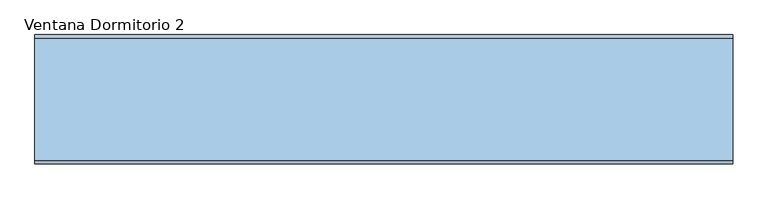
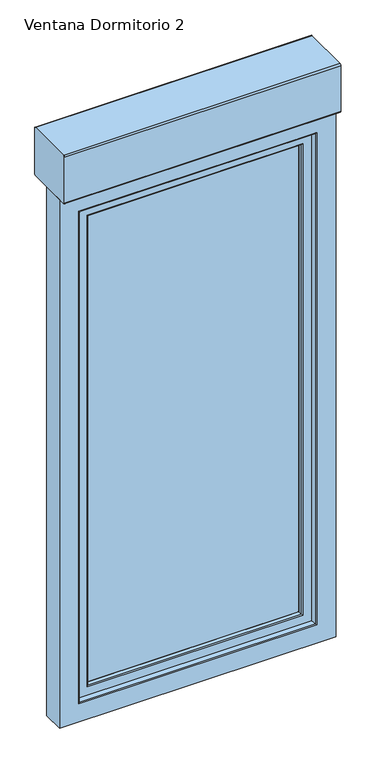
"""IFC4 building model written with IfcOpenShell, lengths in millimetres: window geometry, 2019_ES_Ventana_Replus_re80pvc301_10100_box_1-Hoja_con-Compacto : Ventana Dormitorio 2."""

import ifcopenshell
import ifcopenshell.guid

model = None  # the IFC model being written
_history = None  # IfcOwnerHistory: only IFC2X3 demands one
_inside = {}  # id of a spatial element -> (the spatial element, [elements in it])
_under = {}  # id of a project, library or spatial element -> (it, [spatial elements below it])
_declared = {}  # id of a project -> (the project, [libraries it declares])
_typed = {}  # id of a type object -> (the type object, [elements of that type])
_made_of = {}  # id of a material, layer set ... -> (it, [elements and type objects made of it])


def new_model(schema):
    """Start an empty IFC model of exactly this schema.

    Asked for "IFC4X3", IfcOpenShell would pick the latest addendum, in which some entities
    have other attributes; the version numbers below select the first issue.
    IFC2X3 requires an IfcOwnerHistory on every rooted entity: one is made here for all.
    """
    global model, _history
    if schema == "IFC4X3":
        model = ifcopenshell.file(schema_version=(4, 3, 0, 0))
    else:
        model = ifcopenshell.file(schema=schema)
    _inside.clear()
    _under.clear()
    _declared.clear()
    _typed.clear()
    _made_of.clear()
    _history = None
    if model.schema == "IFC2X3":
        org = make("IfcOrganization", Name="unknown")
        user = make(
            "IfcPersonAndOrganization",
            ThePerson=make("IfcPerson", FamilyName="unknown"),
            TheOrganization=org,
        )
        app = make(
            "IfcApplication",
            ApplicationDeveloper=org,
            Version="unknown",
            ApplicationFullName="unknown",
            ApplicationIdentifier="unknown",
        )
        _history = make(
            "IfcOwnerHistory",
            OwningUser=user,
            OwningApplication=app,
            ChangeAction="ADDED",
            CreationDate=0,
        )
    return model


def make(cls, **values):
    """One entity of the class cls with the attributes given. An attribute that is None is left unset."""
    return model.create_entity(
        cls, **{name: value for name, value in values.items() if value is not None}
    )


def rooted(cls, **values):
    """An entity with a GlobalId (a new one), such as an element, a storey or a relation."""
    return make(cls, GlobalId=ifcopenshell.guid.new(), OwnerHistory=_history, **values)


def si_unit(unit_type, name, prefix=None):
    """IfcSIUnit, for example si_unit("LENGTHUNIT", "METRE", prefix="MILLI")."""
    return make("IfcSIUnit", UnitType=unit_type, Prefix=prefix, Name=name)


def assignment(units):
    """IfcUnitAssignment: the units of a project."""
    return None if units is None else make("IfcUnitAssignment", Units=units)


def point(xyz):
    """IfcCartesianPoint."""
    return None if xyz is None else make("IfcCartesianPoint", Coordinates=xyz)


def direction(xyz):
    """IfcDirection."""
    return None if xyz is None else make("IfcDirection", DirectionRatios=xyz)


def frame(location, z_axis=None, x_axis=None):
    """IfcAxis2Placement3D, a coordinate frame: its origin and axes. An axis left out is left unset."""
    return make(
        "IfcAxis2Placement3D",
        Location=point(location),
        Axis=direction(z_axis),
        RefDirection=direction(x_axis),
    )


def frame_2d(location, x_axis=None):
    """IfcAxis2Placement2D, a coordinate frame in the plane: its origin and x axis."""
    return make(
        "IfcAxis2Placement2D", Location=point(location), RefDirection=direction(x_axis)
    )


def origin():
    """The frame at (0, 0, 0) with its axes left unset."""
    return frame((0.0, 0.0, 0.0))


def place(relative_to, where):
    """IfcLocalPlacement: puts the frame where relative to a parent placement (None: the world)."""
    return make(
        "IfcLocalPlacement", PlacementRelTo=relative_to, RelativePlacement=where
    )


def context(
    kind, dimensions, precision=None, world=None, true_north=None, identifier=None
):
    """IfcGeometricRepresentationContext, for example the 3D "Model" context."""
    return make(
        "IfcGeometricRepresentationContext",
        ContextIdentifier=identifier,
        ContextType=kind,
        CoordinateSpaceDimension=dimensions,
        Precision=precision,
        WorldCoordinateSystem=world,
        TrueNorth=true_north,
    )


def project(units=None, contexts=None):
    """IfcProject with its units and contexts."""
    return rooted(
        "IfcProject",
        Name="project",
        RepresentationContexts=contexts,
        UnitsInContext=assignment(units),
    )


def spatial(cls, under=None, at=None, **own):
    """A site, building, storey or space (cls), placed at a placement, below another one or the project."""
    s = rooted(cls, ObjectPlacement=at, **own)
    if under is not None:
        _under.setdefault(under.id(), (under, []))[1].append(s)
    return s


def polyline(points):
    """IfcPolyline through the points."""
    return make("IfcPolyline", Points=[point(p) for p in points])


def circle_curve(where, radius):
    """IfcCircle in the frame where."""
    return make("IfcCircle", Position=where, Radius=radius)


def ellipse_curve(where, semi_axis1, semi_axis2):
    """IfcEllipse in the frame where."""
    return make(
        "IfcEllipse", Position=where, SemiAxis1=semi_axis1, SemiAxis2=semi_axis2
    )


def trimmed(basis, trim1, trim2, sense, master):
    """IfcTrimmedCurve: the piece of a basis curve between two trims."""
    return make(
        "IfcTrimmedCurve",
        BasisCurve=basis,
        Trim1=trim1,
        Trim2=trim2,
        SenseAgreement=sense,
        MasterRepresentation=master,
    )


def segment(curve, same_sense, transition):
    """IfcCompositeCurveSegment."""
    return make(
        "IfcCompositeCurveSegment",
        Transition=transition,
        SameSense=same_sense,
        ParentCurve=curve,
    )


def composite_curve(segments, self_intersect=None):
    """IfcCompositeCurve: segments joined end to end."""
    return make("IfcCompositeCurve", Segments=segments, SelfIntersect=self_intersect)


def outline(outer, holes=None, kind="AREA"):
    """IfcArbitraryClosedProfileDef: a profile drawn as a closed curve; with holes, ...WithVoids."""
    if holes is None:
        return make("IfcArbitraryClosedProfileDef", ProfileType=kind, OuterCurve=outer)
    return make(
        "IfcArbitraryProfileDefWithVoids",
        ProfileType=kind,
        OuterCurve=outer,
        InnerCurves=holes,
    )


def extrude(swept, where, along, depth):
    """IfcExtrudedAreaSolid: the profile swept, set in the frame where, extruded along a direction by depth."""
    return make(
        "IfcExtrudedAreaSolid",
        SweptArea=swept,
        Position=where,
        ExtrudedDirection=direction(along),
        Depth=depth,
    )


def shape(context_of_items, identifier, shape_type, items):
    """IfcShapeRepresentation: the items that make up one representation, for example the "Body"."""
    return make(
        "IfcShapeRepresentation",
        ContextOfItems=context_of_items,
        RepresentationIdentifier=identifier,
        RepresentationType=shape_type,
        Items=items,
    )


def source(mapping_origin, context_of_items, identifier, shape_type, items):
    """IfcRepresentationMap: a shape defined once, which mapped items show again and again."""
    return make(
        "IfcRepresentationMap",
        MappingOrigin=mapping_origin,
        MappedRepresentation=shape(context_of_items, identifier, shape_type, items),
    )


def transform(
    local_origin,
    x_axis=None,
    y_axis=None,
    z_axis=None,
    scale=None,
    scale2=None,
    scale3=None,
    uniform=True,
):
    """IfcCartesianTransformationOperator3D, or its non-uniform kind. x_axis, y_axis, z_axis: its Axis1, 2, 3."""
    if uniform:
        return make(
            "IfcCartesianTransformationOperator3D",
            Axis1=direction(x_axis),
            Axis2=direction(y_axis),
            LocalOrigin=point(local_origin),
            Scale=scale,
            Axis3=direction(z_axis),
        )
    return make(
        "IfcCartesianTransformationOperator3DnonUniform",
        Axis1=direction(x_axis),
        Axis2=direction(y_axis),
        LocalOrigin=point(local_origin),
        Scale=scale,
        Axis3=direction(z_axis),
        Scale2=scale2,
        Scale3=scale3,
    )


def mapped(mapping_source, mapping_target):
    """IfcMappedItem: shows the shape of a source again, moved by a transform."""
    return make(
        "IfcMappedItem", MappingSource=mapping_source, MappingTarget=mapping_target
    )


def made_of(thing, what):
    """Note that an element or type object is made of a material, layer set ...; save() writes the relation."""
    if what is not None:
        _made_of.setdefault(what.id(), (what, []))[1].append(thing)
    return thing


def element(
    cls,
    number,
    at=None,
    inside=None,
    cuts=None,
    type_object=None,
    material=None,
    context=None,
    identifier="Body",
    shape_type=None,
    held_by="IfcProductDefinitionShape",
    body=None,
    shapes=None,
    **own,
):
    """One element of the class cls, such as IfcWall. Its Tag is "e" and its number.

    at: its placement. inside: the storey or other place that contains it. cuts: it is an
    opening in that element (IfcRelVoidsElement). A single representation is given by context,
    identifier, shape_type and body (its items); several are given by shapes. held_by: the class
    of the entity that holds the representations. save() writes the other relations.
    """
    e = rooted(cls, Tag="e%d" % number, ObjectPlacement=at, **own)
    if body is not None:
        shapes = [shape(context, identifier, shape_type, body)]
    if shapes is not None:
        e.Representation = make(held_by, Representations=shapes)
    if inside is not None:
        _inside.setdefault(inside.id(), (inside, []))[1].append(e)
    if cuts is not None:
        rooted(
            "IfcRelVoidsElement", RelatingBuildingElement=cuts, RelatedOpeningElement=e
        )
    if type_object is not None:
        _typed.setdefault(type_object.id(), (type_object, []))[1].append(e)
    return made_of(e, material)


def aggregate(whole, parts):
    """IfcRelAggregates: a whole, such as a stair, and the parts it consists of."""
    return rooted("IfcRelAggregates", RelatingObject=whole, RelatedObjects=parts)


def save(model, path):
    """Write the relations noted so far, then the file.

    IfcRelAggregates (storeys below a building ...), IfcRelContainedInSpatialStructure (elements
    in a storey), IfcRelDefinesByType, IfcRelAssociatesMaterial and IfcRelDeclares: one each for
    every whole, place, type object, material and project.
    """
    for whole, parts in _under.values():
        aggregate(whole, parts)
    for where, things in _inside.values():
        rooted(
            "IfcRelContainedInSpatialStructure",
            RelatedElements=things,
            RelatingStructure=where,
        )
    for kind, things in _typed.values():
        rooted("IfcRelDefinesByType", RelatedObjects=things, RelatingType=kind)
    for what, things in _made_of.values():
        rooted("IfcRelAssociatesMaterial", RelatedObjects=things, RelatingMaterial=what)
    for by, libraries in _declared.values():
        rooted("IfcRelDeclares", RelatingContext=by, RelatedDefinitions=libraries)
    model.write(path)


def plane_surface(at):
    """IfcPlane: the flat surface through the origin of the frame at, square to its z axis."""
    return make("IfcPlane", Position=at)


def cylinder_surface(at, radius):
    """IfcCylindricalSurface: all points at the distance radius from the z axis of the frame at."""
    return make("IfcCylindricalSurface", Position=at, Radius=radius)


def advanced_brep(points, edges, surfaces, faces):
    """IfcAdvancedBrep: a solid bounded by faces that lie on surfaces and meet in shared edges.

    An edge is (start, end): straight between two places in points (the first is 0);
    or (start, end, curve); or (start, end, curve, False) where it runs against its curve.
    A face is (place in surfaces, loops), or (place, loops, False) where it looks against
    its surface's normal. A loop lists edges by number (the first is 1), with a minus sign
    where the edge is run from its end to its start. The first loop is the outer one.
    """
    corners = [point(p) for p in points]
    vertices = [make("IfcVertexPoint", VertexGeometry=c) for c in corners]
    made = []
    for start, end, *more in edges:
        made.append(
            make(
                "IfcEdgeCurve",
                EdgeStart=vertices[start],
                EdgeEnd=vertices[end],
                EdgeGeometry=more[0] if more else make("IfcPolyline", Points=[corners[start], corners[end]]),
                SameSense=more[1] if len(more) > 1 else True,
            )
        )
    hull = []
    for where, loops, *sense in faces:
        bounds = []
        for j, loop in enumerate(loops):
            ring = [make("IfcOrientedEdge", EdgeElement=made[abs(k) - 1], Orientation=k > 0) for k in loop]
            bounds.append(
                make(
                    "IfcFaceOuterBound" if j == 0 else "IfcFaceBound",
                    Bound=make("IfcEdgeLoop", EdgeList=ring),
                    Orientation=True,
                )
            )
        hull.append(make("IfcAdvancedFace", Bounds=bounds, FaceSurface=surfaces[where], SameSense=sense[0] if sense else True))
    return make("IfcAdvancedBrep", Outer=make("IfcClosedShell", CfsFaces=hull))


def ventana_dormitorio_2_fe78aa6e(model_context):
    return source(origin(), model_context, "Body", "SolidModel", [
        extrude(outline(composite_curve([segment(trimmed(circle_curve(frame_2d((-55.0, 2835.0)), 5.0), [point((-55.0, 2830.0))], [point((-60.0, 2835.0))], False, "CARTESIAN"), True, "CONTINUOUS"), segment(polyline([(-60.0, 2835.0), (-60.0, 3010.0)]), True, "CONTINUOUS"), segment(trimmed(circle_curve(frame_2d((-55.0, 3010.0)), 5.0), [point((-60.0, 3010.0))], [point((-55.0, 3015.0))], False, "CARTESIAN"), True, "CONTINUOUS"), segment(polyline([(-55.0, 3015.0), (120.0, 3015.0)]), True, "CONTINUOUS"), segment(trimmed(circle_curve(frame_2d((120.0, 3010.0)), 5.0), [point((120.0, 3015.0))], [point((125.0, 3010.0))], False, "CARTESIAN"), True, "CONTINUOUS"), segment(polyline([(125.0, 3010.0), (125.0, 2835.0)]), True, "CONTINUOUS"), segment(trimmed(circle_curve(frame_2d((120.0, 2835.0)), 5.0), [point((125.0, 2835.0))], [point((120.0, 2830.0))], False, "CARTESIAN"), True, "CONTINUOUS"), segment(polyline([(120.0, 2830.0), (-55.0, 2830.0)]), True, "CONTINUOUS")], self_intersect=False)), frame((-500.0, 0.0, 0.0), z_axis=(1.0, 0.0, 0.0), x_axis=(0.0, 1.0, 0.0)), (0.0, 0.0, 1.0), 1000.0),
        extrude(outline(polyline([(78.4999991, 1470.0), (118.4999991, 1470.0), (118.4999991, 1360.0), (98.4999991, 1360.0), (98.4999991, 1450.0), (78.4999991, 1450.0), (78.4999991, 1470.0)])), frame((-434.1999993, 0.0, 0.0), z_axis=(1.0, 0.0, 0.0), x_axis=(0.0, 1.0, 0.0)), (0.0, 0.0, 1.0), 12.0),
        extrude(outline(polyline([(-413.9687607, 78.4999991), (-413.9687607, 68.4999991), (-442.4312378, 68.4999991), (-442.4312378, 78.4999991), (-413.9687607, 78.4999991)])), frame((0.0, 0.0, 1435.217127), z_axis=(0.0, 0.0, 1.0), x_axis=(1.0, 0.0, 0.0)), (0.0, 0.0, 1.0), 49.565746),
        extrude(outline(polyline([(909.8, 397.1999993), (2727.2, 397.1999993), (2727.2, -397.1999993), (909.8, -397.1999993), (909.8, 397.1999993)]), holes=[polyline([(2719.2, 389.1999993), (917.8, 389.1999993), (917.8, -389.1999993), (2719.2, -389.1999993), (2719.2, 389.1999993)])]), frame((0.0, 10.9999999, 0.0), z_axis=(0.0, 1.0, 0.0), x_axis=(0.0, 0.0, 1.0)), (0.0, 0.0, 1.0), 16.0),
        extrude(outline(polyline([(909.8131934, 397.1868058), (2727.1868066, 397.1868058), (2727.1868066, -397.1868058), (909.8131934, -397.1868058), (909.8131934, 397.1868058)]), holes=[polyline([(2719.2, 389.1999993), (917.8, 389.1999993), (917.8, -389.1999993), (2719.2, -389.1999993), (2719.2, 389.1999993)])]), frame((0.0, 31.0000001, 0.0), z_axis=(0.0, 1.0, 0.0), x_axis=(0.0, 0.0, 1.0)), (0.0, 0.0, 1.0), 16.0),
        extrude(outline(polyline([(397.1999993, 6.9999997), (-397.1999993, 6.9999997), (-397.1999993, 10.9999999), (397.1999993, 10.9999999), (397.1999993, 6.9999997)])), frame((0.0, 0.0, 903.7946451), z_axis=(0.0, 0.0, 1.0), x_axis=(1.0, 0.0, 0.0)), (0.0, 0.0, 1.0), 1829.4053549),
        extrude(outline(polyline([(397.1999993, 26.9999999), (-397.1999993, 26.9999999), (-397.1999993, 31.0000001), (397.1999993, 31.0000001), (397.1999993, 26.9999999)])), frame((0.0, 0.0, 903.7946451), z_axis=(0.0, 0.0, 1.0), x_axis=(1.0, 0.0, 0.0)), (0.0, 0.0, 1.0), 1829.4053549),
        extrude(outline(polyline([(397.1999993, 47.0000001), (-397.1999993, 47.0000001), (-397.1999993, 51.0000003), (397.1999993, 51.0000003), (397.1999993, 47.0000001)])), frame((0.0, 0.0, 903.7946451), z_axis=(0.0, 0.0, 1.0), x_axis=(1.0, 0.0, 0.0)), (0.0, 0.0, 1.0), 1829.4053549),
        advanced_brep(
        [(387.2913171, -9.2764571, 2717.2913178), (387.2913171, -9.2764571, 922.7086822), (390.1890946, -11.5, 919.8109047), (390.1890946, -11.5, 2720.1890953), (430.1999993, -11.5, 879.8), (430.1999993, -11.5, 2760.2), (-430.1999993, -11.5, 2760.2), (-430.1999993, -11.5, 879.8), (-390.1890946, -11.5, 919.8109047), (-390.1890946, -11.5, 2720.1890953), (-387.2913171, -9.2764571, 922.7086822), (384.1757968, 2.3508228, 2714.1757976), (384.1757968, 2.3508228, 925.8242024), (-384.1757968, 2.3508228, 925.8242024), (384.6739305, 3.0000033, 2714.6739313), (384.6739305, 3.0000033, 925.3260687), (-384.6739305, 3.0000033, 925.3260687), (391.1999993, 3.0000033, 2721.2), (391.1999993, 3.0000033, 918.8), (-391.1999993, 3.0000033, 918.8), (-391.1999993, 3.0000033, 2721.2), (-384.6739305, 3.0000033, 2714.6739313), (391.1999993, 6.9999997, 2721.2), (391.1999993, 6.9999997, 918.8), (-391.1999993, 6.9999997, 918.8), (411.8162192, 6.9999997, 2741.8162199), (411.8162192, 6.9999997, 898.1837801), (-411.8162192, 6.9999997, 898.1837801), (-411.8162192, 6.9999997, 2741.8162199), (-391.1999993, 6.9999997, 2721.2), (409.1999993, 25.6153717, 2739.2), (409.1999993, 25.6153717, 900.8), (-409.1999993, 25.6153717, 900.8), (409.1999993, 56.4999995, 2739.2), (409.1999993, 56.4999995, 900.8), (-409.1999993, 56.4999995, 900.8), (-409.1999993, 56.4999995, 2739.2), (397.1999993, 56.4999995, 2727.2), (397.1999993, 56.4999995, 912.8), (-397.1999993, 56.4999995, 912.8), (-397.1999993, 56.4999995, 2727.2), (397.1999993, 51.0000003, 2727.2), (397.1999993, 51.0000003, 912.8), (-397.1999993, 51.0000003, 912.8), (-397.1999993, 51.0000003, 2727.2), (386.007687, 51.0000003, 2716.0076877), (386.007687, 51.0000003, 923.9923123), (-386.007687, 51.0000003, 923.9923123), (-386.007687, 51.0000003, 2716.0076877), (385.4940999, 51.6693201, 2715.4941006), (385.4940999, 51.6693201, 924.5058994), (-385.4940999, 51.6693201, 924.5058994), (388.8993918, 64.3780426, 2718.8993925), (388.8993918, 64.3780426, 921.1006075), (-388.8993918, 64.3780426, 921.1006075), (392.6234971, 67.3403297, 2722.6234978), (392.6234971, 67.3403297, 917.3765022), (-392.6234971, 67.3403297, 917.3765022), (405.6488427, 67.7951848, 2735.6488434), (405.6488427, 67.7951848, 904.3511566), (-405.6488427, 67.7951848, 904.3511566), (406.1999993, 67.2629391, 2736.2), (406.1999993, 67.2629391, 903.8), (-406.1999993, 67.2629391, 903.8), (407.4370593, 68.4999991, 2737.43706), (407.4370593, 68.4999991, 902.56294), (-407.4370593, 68.4999991, 902.56294), (460.1999993, 68.4999991, 2790.2), (460.1999993, 68.4999991, 849.8), (-460.1999993, 68.4999991, 849.8), (-460.1999993, 68.4999991, 2790.2), (-407.4370593, 68.4999991, 2737.43706), (463.1999993, 65.4999991, 2793.2), (463.1999993, 65.4999991, 846.8), (-463.1999993, 65.4999991, 846.8), (463.1999993, 50.0, 2793.2), (463.1999993, 50.0, 846.8), (-463.1999993, 50.0, 846.8), (-463.1999993, 50.0, 2793.2), (443.1999993, 50.0, 2773.2), (443.1999993, 50.0, 866.8), (-443.1999993, 50.0, 866.8), (-443.1999993, 50.0, 2773.2), (443.1999993, 11.9999991, 2773.2), (443.1999993, 11.9999991, 866.8), (-443.1999993, 11.9999991, 866.8), (-443.1999993, 11.9999991, 2773.2), (430.1999993, 11.9999991, 2760.2), (430.1999993, 11.9999991, 879.8), (-430.1999993, 11.9999991, 879.8), (-430.1999993, 11.9999991, 2760.2), (-387.2913171, -9.2764571, 2717.2913178), (-384.1757968, 2.3508228, 2714.1757976), (-409.1999993, 25.6153717, 2739.2), (-385.4940999, 51.6693201, 2715.4941006), (-388.8993918, 64.3780426, 2718.8993925), (-392.6234971, 67.3403297, 2722.6234978), (-405.6488427, 67.7951848, 2735.6488434), (-406.1999993, 67.2629391, 2736.2), (-463.1999993, 65.4999991, 2793.2)],
        [
            (0, 1),
            (1, 2, ellipse_curve(frame((390.1890946, -8.5, 919.8109047), z_axis=(0.7071067811865475, 0.0, 0.7071067811865475), x_axis=(-0.7071067811865474, 0.0, 0.7071067811865476)), 4.2426407, 3.0)),
            (2, 3),
            (3, 0, ellipse_curve(frame((390.1890946, -8.5, 2720.1890953), z_axis=(0.7071067811865475, 0.0, -0.7071067811865475), x_axis=(0.7071067811865474, 0.0, 0.7071067811865476)), 4.2426407, 3.0)),
            (4, 5),
            (5, 6),
            (6, 7),
            (7, 4),
            (2, 8),
            (8, 9),
            (9, 3),
            (1, 10),
            (10, 8, ellipse_curve(frame((-390.1890946, -8.5, 919.8109047), z_axis=(0.7071067811865475, 0.0, -0.7071067811865475), x_axis=(0.7071067811865476, 0.0, 0.7071067811865474)), 4.2426407, 3.0)),
            (11, 12),
            (12, 1),
            (0, 11),
            (12, 13),
            (13, 10),
            (14, 15),
            (15, 12, ellipse_curve(frame((384.6739305, 2.4842973, 925.3260687), z_axis=(0.7071067811865475, 0.0, 0.7071067811865475), x_axis=(-0.7071067811865474, 0.0, 0.7071067811865476)), 0.7293184, 0.515706)),
            (11, 14, ellipse_curve(frame((384.6739305, 2.4842973, 2714.6739313), z_axis=(0.7071067811865475, 0.0, -0.7071067811865475), x_axis=(0.7071067811865474, 0.0, 0.7071067811865476)), 0.7293184, 0.515706)),
            (15, 16),
            (16, 13, ellipse_curve(frame((-384.6739305, 2.4842973, 925.3260687), z_axis=(0.7071067811865475, 0.0, -0.7071067811865475), x_axis=(0.7071067811865476, 0.0, 0.7071067811865474)), 0.7293184, 0.515706)),
            (17, 18),
            (18, 19),
            (19, 20),
            (20, 17),
            (14, 21),
            (21, 16),
            (22, 23),
            (23, 18),
            (17, 22),
            (23, 24),
            (24, 19),
            (25, 26),
            (26, 27),
            (27, 28),
            (28, 25),
            (22, 29),
            (29, 24),
            (30, 31),
            (31, 26),
            (25, 30),
            (31, 32),
            (32, 27),
            (33, 34),
            (34, 31),
            (30, 33),
            (34, 35),
            (35, 32),
            (33, 36),
            (36, 35),
            (37, 38),
            (38, 39),
            (39, 40),
            (40, 37),
            (41, 42),
            (42, 38),
            (37, 41),
            (42, 43),
            (43, 39),
            (41, 44),
            (44, 43),
            (45, 46),
            (46, 47),
            (47, 48),
            (48, 45),
            (49, 50),
            (50, 46, ellipse_curve(frame((386.007687, 51.5317048, 923.9923123), z_axis=(0.7071067811865475, 0.0, 0.7071067811865475), x_axis=(-0.7071067811865474, 0.0, 0.7071067811865476)), 0.7519437, 0.5317045)),
            (45, 49, ellipse_curve(frame((386.007687, 51.5317048, 2716.0076877), z_axis=(0.7071067811865475, 0.0, -0.7071067811865475), x_axis=(0.7071067811865474, 0.0, 0.7071067811865476)), 0.7519437, 0.5317045)),
            (50, 51),
            (51, 47, ellipse_curve(frame((-386.007687, 51.5317048, 923.9923123), z_axis=(0.7071067811865475, 0.0, -0.7071067811865475), x_axis=(0.7071067811865476, 0.0, 0.7071067811865474)), 0.7519437, 0.5317045)),
            (52, 53),
            (53, 50),
            (49, 52),
            (53, 54),
            (54, 51),
            (55, 56),
            (56, 53, ellipse_curve(frame((392.7630951, 63.3427664, 917.2369042), z_axis=(0.7071067811865475, 0.0, 0.7071067811865475), x_axis=(-0.7071067811865474, 0.0, 0.7071067811865476)), 5.6568542, 4.0)),
            (52, 55, ellipse_curve(frame((392.7630951, 63.3427664, 2722.7630958), z_axis=(0.7071067811865475, 0.0, -0.7071067811865475), x_axis=(0.7071067811865474, 0.0, 0.7071067811865476)), 5.6568542, 4.0)),
            (56, 57),
            (57, 54, ellipse_curve(frame((-392.7630951, 63.3427664, 917.2369042), z_axis=(0.7071067811865475, 0.0, -0.7071067811865475), x_axis=(0.7071067811865476, 0.0, 0.7071067811865474)), 5.6568542, 4.0)),
            (58, 59),
            (59, 56),
            (55, 58),
            (59, 60),
            (60, 57),
            (61, 62),
            (62, 59, ellipse_curve(frame((405.6674291, 67.2629391, 904.3325701), z_axis=(0.7071067811865475, 0.0, 0.7071067811865475), x_axis=(-0.7071067811865474, 0.0, 0.7071067811865476)), 0.7531679, 0.5325701)),
            (58, 61, ellipse_curve(frame((405.6674291, 67.2629391, 2735.6674299), z_axis=(0.7071067811865475, 0.0, -0.7071067811865475), x_axis=(0.7071067811865474, 0.0, 0.7071067811865476)), 0.7531679, 0.5325701)),
            (62, 63),
            (63, 60, ellipse_curve(frame((-405.6674291, 67.2629391, 904.3325701), z_axis=(0.7071067811865475, 0.0, -0.7071067811865475), x_axis=(0.7071067811865476, 0.0, 0.7071067811865474)), 0.7531679, 0.5325701)),
            (64, 65),
            (65, 62, ellipse_curve(frame((407.4370593, 67.2629391, 902.56294), z_axis=(0.7071067811865475, 0.0, 0.7071067811865475), x_axis=(-0.7071067811865474, 0.0, 0.7071067811865476)), 1.7494671, 1.23706)),
            (61, 64, ellipse_curve(frame((407.4370593, 67.2629391, 2737.43706), z_axis=(0.7071067811865475, 0.0, -0.7071067811865475), x_axis=(0.7071067811865474, 0.0, 0.7071067811865476)), 1.7494671, 1.23706)),
            (65, 66),
            (66, 63, ellipse_curve(frame((-407.4370593, 67.2629391, 902.56294), z_axis=(0.7071067811865475, 0.0, -0.7071067811865475), x_axis=(0.7071067811865476, 0.0, 0.7071067811865474)), 1.7494671, 1.23706)),
            (67, 68),
            (68, 69),
            (69, 70),
            (70, 67),
            (64, 71),
            (71, 66),
            (72, 73),
            (73, 68, ellipse_curve(frame((460.1999993, 65.4999991, 849.8), z_axis=(0.7071067811865475, 0.0, 0.7071067811865475), x_axis=(-0.7071067811865474, 0.0, 0.7071067811865476)), 4.2426407, 3.0)),
            (67, 72, ellipse_curve(frame((460.1999993, 65.4999991, 2790.2), z_axis=(0.7071067811865475, 0.0, -0.7071067811865475), x_axis=(0.7071067811865474, 0.0, 0.7071067811865476)), 4.2426407, 3.0)),
            (73, 74),
            (74, 69, ellipse_curve(frame((-460.1999993, 65.4999991, 849.8), z_axis=(0.7071067811865475, 0.0, -0.7071067811865475), x_axis=(0.7071067811865476, 0.0, 0.7071067811865474)), 4.2426407, 3.0)),
            (75, 76),
            (76, 73),
            (72, 75),
            (76, 77),
            (77, 74),
            (75, 78),
            (78, 77),
            (79, 80),
            (80, 81),
            (81, 82),
            (82, 79),
            (79, 83),
            (83, 84),
            (84, 80),
            (84, 85),
            (85, 81),
            (83, 86),
            (86, 85),
            (87, 88),
            (88, 89),
            (89, 90),
            (90, 87),
            (87, 5),
            (4, 88),
            (7, 89),
            (10, 91),
            (91, 9, ellipse_curve(frame((-390.1890946, -8.5, 2720.1890953), z_axis=(-0.7071067811865475, 0.0, -0.7071067811865475), x_axis=(0.7071067811865474, 0.0, -0.7071067811865476)), 4.2426407, 3.0)),
            (13, 92),
            (92, 91),
            (21, 92, ellipse_curve(frame((-384.6739305, 2.4842973, 2714.6739313), z_axis=(-0.7071067811865475, 0.0, -0.7071067811865475), x_axis=(0.7071067811865474, 0.0, -0.7071067811865476)), 0.7293184, 0.515706)),
            (29, 20),
            (32, 93),
            (93, 28),
            (36, 93),
            (44, 40),
            (51, 94),
            (94, 48, ellipse_curve(frame((-386.007687, 51.5317048, 2716.0076877), z_axis=(-0.7071067811865475, 0.0, -0.7071067811865475), x_axis=(0.7071067811865474, 0.0, -0.7071067811865476)), 0.7519437, 0.5317045)),
            (54, 95),
            (95, 94),
            (57, 96),
            (96, 95, ellipse_curve(frame((-392.7630951, 63.3427664, 2722.7630958), z_axis=(-0.7071067811865475, 0.0, -0.7071067811865475), x_axis=(0.7071067811865474, 0.0, -0.7071067811865476)), 5.6568542, 4.0)),
            (60, 97),
            (97, 96),
            (63, 98),
            (98, 97, ellipse_curve(frame((-405.6674291, 67.2629391, 2735.6674299), z_axis=(-0.7071067811865475, 0.0, -0.7071067811865475), x_axis=(0.7071067811865474, 0.0, -0.7071067811865476)), 0.7531679, 0.5325701)),
            (71, 98, ellipse_curve(frame((-407.4370593, 67.2629391, 2737.43706), z_axis=(-0.7071067811865475, 0.0, -0.7071067811865475), x_axis=(0.7071067811865474, 0.0, -0.7071067811865476)), 1.7494671, 1.23706)),
            (74, 99),
            (99, 70, ellipse_curve(frame((-460.1999993, 65.4999991, 2790.2), z_axis=(-0.7071067811865475, 0.0, -0.7071067811865475), x_axis=(0.7071067811865474, 0.0, -0.7071067811865476)), 4.2426407, 3.0)),
            (78, 99),
            (86, 82),
            (6, 90),
            (91, 0),
            (92, 11),
            (93, 30),
            (94, 49),
            (95, 52),
            (96, 55),
            (97, 58),
            (98, 61),
            (99, 72),
        ],
        [
            cylinder_surface(frame((390.1890946, -8.5, 2793.2), z_axis=(0.0, 0.0, 1.0), x_axis=(-1.0, 0.0, 0.0)), 3.0),
            plane_surface(frame((-430.1999993, -11.5, 2760.2), z_axis=(0.0, -1.0, 0.0), x_axis=(1.0, 0.0, 0.0))),
            cylinder_surface(frame((463.1999993, -8.5, 919.8109047), z_axis=(1.0, 0.0, 0.0), x_axis=(0.0, 0.0, 1.0)), 3.0),
            plane_surface(frame((387.2913171, -9.2764571, 2717.2913178), z_axis=(-0.9659258263570549, -0.2588190448487916, 0.0), x_axis=(0.0, 0.0, -1.0))),
            plane_surface(frame((387.2913171, -9.2764571, 922.7086822), z_axis=(0.0, -0.2588190448487885, 0.9659258263570558), x_axis=(-1.0, 0.0, 0.0))),
            cylinder_surface(frame((384.6739305, 2.4842973, 2793.2), z_axis=(0.0, 0.0, 1.0), x_axis=(-1.0, 0.0, 0.0)), 0.515706),
            cylinder_surface(frame((463.1999993, 2.4842973, 925.3260687), z_axis=(1.0, 0.0, 0.0), x_axis=(0.0, 0.0, 1.0)), 0.515706),
            plane_surface(frame((-384.6739305, 3.0000033, 2714.6739313), z_axis=(0.0, 1.0, 0.0), x_axis=(1.0, 0.0, 0.0))),
            plane_surface(frame((391.1999993, 3.0000033, 2721.2), z_axis=(-1.0, 0.0, 0.0), x_axis=(0.0, 0.0, -1.0))),
            plane_surface(frame((391.1999993, 3.0000033, 918.8), z_axis=(0.0, 0.0, 1.0), x_axis=(-1.0, 0.0, 0.0))),
            plane_surface(frame((-391.1999993, 6.9999997, 2721.2), z_axis=(0.0, 1.0, 0.0), x_axis=(1.0, 0.0, 0.0))),
            plane_surface(frame((411.8162192, 6.9999997, 2741.8162199), z_axis=(-0.9902680687415736, -0.13917310096004265, 0.0), x_axis=(0.0, 0.0, -1.0))),
            plane_surface(frame((411.8162192, 6.9999997, 898.1837801), z_axis=(0.0, -0.13917310096003946, 0.990268068741574), x_axis=(-1.0, 0.0, 0.0))),
            plane_surface(frame((409.1999993, 25.6153717, 2739.2), z_axis=(-1.0, 0.0, 0.0), x_axis=(0.0, 0.0, -1.0))),
            plane_surface(frame((409.1999993, 25.6153717, 900.8), z_axis=(0.0, 0.0, 1.0), x_axis=(-1.0, 0.0, 0.0))),
            plane_surface(frame((-409.1999993, 56.4999995, 2739.2), z_axis=(0.0, -1.0, 0.0), x_axis=(1.0, 0.0, 0.0))),
            plane_surface(frame((397.1999993, 56.4999995, 2727.2), z_axis=(1.0, 0.0, 0.0), x_axis=(0.0, 0.0, -1.0))),
            plane_surface(frame((397.1999993, 56.4999995, 912.8), z_axis=(0.0, 0.0, -1.0), x_axis=(-1.0, 0.0, 0.0))),
            plane_surface(frame((-397.1999993, 51.0000003, 2727.2), z_axis=(0.0, -1.0, 0.0), x_axis=(1.0, 0.0, 0.0))),
            cylinder_surface(frame((386.007687, 51.5317048, 2793.2), z_axis=(0.0, 0.0, 1.0), x_axis=(-1.0, 0.0, 0.0)), 0.5317045),
            cylinder_surface(frame((463.1999993, 51.5317048, 923.9923123), z_axis=(1.0, 0.0, 0.0), x_axis=(0.0, 0.0, 1.0)), 0.5317045),
            plane_surface(frame((385.4940999, 51.6693201, 2715.4941006), z_axis=(-0.9659258262890666, 0.2588190451025272, 0.0), x_axis=(0.0, 0.0, -1.0))),
            plane_surface(frame((385.4940999, 51.6693201, 924.5058994), z_axis=(0.0, 0.2588190451025303, 0.9659258262890658), x_axis=(-1.0, 0.0, 0.0))),
            cylinder_surface(frame((392.7630951, 63.3427664, 2793.2), z_axis=(0.0, 0.0, 1.0), x_axis=(-1.0, 0.0, 0.0)), 4.0),
            cylinder_surface(frame((463.1999993, 63.3427664, 917.2369042), z_axis=(1.0, 0.0, 0.0), x_axis=(0.0, 0.0, 1.0)), 4.0),
            plane_surface(frame((392.6234971, 67.3403297, 2722.6234978), z_axis=(-0.034899496702507804, 0.9993908270190955, 0.0), x_axis=(0.0, 0.0, -1.0))),
            plane_surface(frame((392.6234971, 67.3403297, 917.3765022), z_axis=(0.0, 0.9993908270190957, 0.03489949670250457), x_axis=(-1.0, 0.0, 0.0))),
            cylinder_surface(frame((405.6674291, 67.2629391, 2793.2), z_axis=(0.0, 0.0, 1.0), x_axis=(-1.0, 0.0, 0.0)), 0.5325701),
            cylinder_surface(frame((463.1999993, 67.2629391, 904.3325701), z_axis=(1.0, 0.0, 0.0), x_axis=(0.0, 0.0, 1.0)), 0.5325701),
            cylinder_surface(frame((407.4370593, 67.2629391, 2793.2), z_axis=(0.0, 0.0, 1.0), x_axis=(-1.0, 0.0, 0.0)), 1.23706),
            cylinder_surface(frame((463.1999993, 67.2629391, 902.56294), z_axis=(1.0, 0.0, 0.0), x_axis=(0.0, 0.0, 1.0)), 1.23706),
            plane_surface(frame((-407.4370593, 68.4999991, 2737.43706), z_axis=(0.0, 1.0, 0.0), x_axis=(1.0, 0.0, 0.0))),
            cylinder_surface(frame((460.1999993, 65.4999991, 2793.2), z_axis=(0.0, 0.0, 1.0), x_axis=(-1.0, 0.0, 0.0)), 3.0),
            cylinder_surface(frame((463.1999993, 65.4999991, 849.8), z_axis=(1.0, 0.0, 0.0), x_axis=(0.0, 0.0, 1.0)), 3.0),
            plane_surface(frame((463.1999993, 65.4999991, 2793.2), z_axis=(1.0, 0.0, 0.0), x_axis=(0.0, 0.0, -1.0))),
            plane_surface(frame((463.1999993, 65.4999991, 846.8), z_axis=(0.0, 0.0, -1.0), x_axis=(-1.0, 0.0, 0.0))),
            plane_surface(frame((-459.2000019, 50.0, 2789.2000027), z_axis=(0.0, -1.0, 0.0), x_axis=(1.0, 0.0, 0.0))),
            plane_surface(frame((443.1999993, 45.0999991, 2773.2), z_axis=(1.0, 0.0, 0.0), x_axis=(0.0, 0.0, -1.0))),
            plane_surface(frame((443.1999993, 45.0999991, 866.8), z_axis=(0.0, 0.0, -1.0), x_axis=(-1.0, 0.0, 0.0))),
            plane_surface(frame((-435.7000002, 11.9999991, 2765.7000009), z_axis=(0.0, -1.0, 0.0), x_axis=(1.0, 0.0, 0.0))),
            plane_surface(frame((430.1999993, 1.4999991, 2760.2), z_axis=(1.0, 0.0, 0.0), x_axis=(0.0, 0.0, -1.0))),
            plane_surface(frame((430.1999993, 1.4999991, 879.8), z_axis=(0.0, 0.0, -1.0), x_axis=(-1.0, 0.0, 0.0))),
            cylinder_surface(frame((-390.1890946, -8.5, 846.8), z_axis=(0.0, 0.0, -1.0), x_axis=(1.0, 0.0, 0.0)), 3.0),
            plane_surface(frame((-387.2913171, -9.2764571, 922.7086822), z_axis=(0.9659258263570565, -0.2588190448487853, 0.0), x_axis=(0.0, 0.0, 1.0))),
            cylinder_surface(frame((-384.6739305, 2.4842973, 846.8), z_axis=(0.0, 0.0, -1.0), x_axis=(1.0, 0.0, 0.0)), 0.515706),
            plane_surface(frame((-391.1999993, 3.0000033, 918.8), z_axis=(1.0, 0.0, 0.0), x_axis=(0.0, 0.0, 1.0))),
            plane_surface(frame((-411.8162192, 6.9999997, 898.1837801), z_axis=(0.9902680687415745, -0.13917310096003627, 0.0), x_axis=(0.0, 0.0, 1.0))),
            plane_surface(frame((-409.1999993, 25.6153717, 900.8), z_axis=(1.0, 0.0, 0.0), x_axis=(0.0, 0.0, 1.0))),
            plane_surface(frame((-397.1999993, 56.4999995, 912.8), z_axis=(-1.0, 0.0, 0.0), x_axis=(0.0, 0.0, 1.0))),
            cylinder_surface(frame((-386.007687, 51.5317048, 846.8), z_axis=(0.0, 0.0, -1.0), x_axis=(1.0, 0.0, 0.0)), 0.5317045),
            plane_surface(frame((-385.4940999, 51.6693201, 924.5058994), z_axis=(0.9659258262890649, 0.2588190451025334, 0.0), x_axis=(0.0, 0.0, 1.0))),
            cylinder_surface(frame((-392.7630951, 63.3427664, 846.8), z_axis=(0.0, 0.0, -1.0), x_axis=(1.0, 0.0, 0.0)), 4.0),
            plane_surface(frame((-392.6234971, 67.3403297, 917.3765022), z_axis=(0.03489949670250134, 0.9993908270190958, 0.0), x_axis=(0.0, 0.0, 1.0))),
            cylinder_surface(frame((-405.6674291, 67.2629391, 846.8), z_axis=(0.0, 0.0, -1.0), x_axis=(1.0, 0.0, 0.0)), 0.5325701),
            cylinder_surface(frame((-407.4370593, 67.2629391, 846.8), z_axis=(0.0, 0.0, -1.0), x_axis=(1.0, 0.0, 0.0)), 1.23706),
            cylinder_surface(frame((-460.1999993, 65.4999991, 846.8), z_axis=(0.0, 0.0, -1.0), x_axis=(1.0, 0.0, 0.0)), 3.0),
            plane_surface(frame((-463.1999993, 65.4999991, 846.8), z_axis=(-1.0, 0.0, 0.0), x_axis=(0.0, 0.0, 1.0))),
            plane_surface(frame((-443.1999993, 45.0999991, 866.8), z_axis=(-1.0, 0.0, 0.0), x_axis=(0.0, 0.0, 1.0))),
            plane_surface(frame((-430.1999993, 1.4999991, 879.8), z_axis=(-1.0, 0.0, 0.0), x_axis=(0.0, 0.0, 1.0))),
            cylinder_surface(frame((-463.1999993, -8.5, 2720.1890953), z_axis=(-1.0, 0.0, 0.0), x_axis=(0.0, 0.0, -1.0)), 3.0),
            plane_surface(frame((-387.2913171, -9.2764571, 2717.2913178), z_axis=(0.0, -0.2588190448487885, -0.9659258263570557), x_axis=(1.0, 0.0, 0.0))),
            cylinder_surface(frame((-463.1999993, 2.4842973, 2714.6739313), z_axis=(-1.0, 0.0, 0.0), x_axis=(0.0, 0.0, -1.0)), 0.515706),
            plane_surface(frame((-391.1999993, 3.0000033, 2721.2), z_axis=(0.0, 0.0, -1.0), x_axis=(1.0, 0.0, 0.0))),
            plane_surface(frame((-411.8162192, 6.9999997, 2741.8162199), z_axis=(0.0, -0.13917310096003946, -0.990268068741574), x_axis=(1.0, 0.0, 0.0))),
            plane_surface(frame((-409.1999993, 25.6153717, 2739.2), z_axis=(0.0, 0.0, -1.0), x_axis=(1.0, 0.0, 0.0))),
            plane_surface(frame((-397.1999993, 56.4999995, 2727.2), z_axis=(0.0, 0.0, 1.0), x_axis=(1.0, 0.0, 0.0))),
            cylinder_surface(frame((-463.1999993, 51.5317048, 2716.0076877), z_axis=(-1.0, 0.0, 0.0), x_axis=(0.0, 0.0, -1.0)), 0.5317045),
            plane_surface(frame((-385.4940999, 51.6693201, 2715.4941006), z_axis=(0.0, 0.2588190451025303, -0.9659258262890658), x_axis=(1.0, 0.0, 0.0))),
            cylinder_surface(frame((-463.1999993, 63.3427664, 2722.7630958), z_axis=(-1.0, 0.0, 0.0), x_axis=(0.0, 0.0, -1.0)), 4.0),
            plane_surface(frame((-392.6234971, 67.3403297, 2722.6234978), z_axis=(0.0, 0.9993908270190957, -0.03489949670250457), x_axis=(1.0, 0.0, 0.0))),
            cylinder_surface(frame((-463.1999993, 67.2629391, 2735.6674299), z_axis=(-1.0, 0.0, 0.0), x_axis=(0.0, 0.0, -1.0)), 0.5325701),
            cylinder_surface(frame((-463.1999993, 67.2629391, 2737.43706), z_axis=(-1.0, 0.0, 0.0), x_axis=(0.0, 0.0, -1.0)), 1.23706),
            cylinder_surface(frame((-463.1999993, 65.4999991, 2790.2), z_axis=(-1.0, 0.0, 0.0), x_axis=(0.0, 0.0, -1.0)), 3.0),
            plane_surface(frame((-463.1999993, 65.4999991, 2793.2), z_axis=(0.0, 0.0, 1.0), x_axis=(1.0, 0.0, 0.0))),
            plane_surface(frame((-443.1999993, 45.0999991, 2773.2), z_axis=(0.0, 0.0, 1.0), x_axis=(1.0, 0.0, 0.0))),
            plane_surface(frame((-430.1999993, 1.4999991, 2760.2), z_axis=(0.0, 0.0, 1.0), x_axis=(1.0, 0.0, 0.0))),
        ],
        [
            (0, [[1, 2, 3, 4]]),
            (1, [[5, 6, 7, 8], [-3, 9, 10, 11]]),
            (2, [[12, 13, -9, -2]]),
            (3, [[14, 15, -1, 16]]),
            (4, [[17, 18, -12, -15]]),
            (5, [[19, 20, -14, 21]]),
            (6, [[22, 23, -17, -20]]),
            (7, [[24, 25, 26, 27], [-19, 28, 29, -22]]),
            (8, [[30, 31, -24, 32]]),
            (9, [[33, 34, -25, -31]]),
            (10, [[35, 36, 37, 38], [-30, 39, 40, -33]]),
            (11, [[41, 42, -35, 43]]),
            (12, [[44, 45, -36, -42]]),
            (13, [[46, 47, -41, 48]]),
            (14, [[49, 50, -44, -47]]),
            (15, [[-46, 51, 52, -49], [53, 54, 55, 56]]),
            (16, [[57, 58, -53, 59]]),
            (17, [[60, 61, -54, -58]]),
            (18, [[-57, 62, 63, -60], [64, 65, 66, 67]]),
            (19, [[68, 69, -64, 70]]),
            (20, [[71, 72, -65, -69]]),
            (21, [[73, 74, -68, 75]]),
            (22, [[76, 77, -71, -74]]),
            (23, [[78, 79, -73, 80]]),
            (24, [[81, 82, -76, -79]]),
            (25, [[83, 84, -78, 85]]),
            (26, [[86, 87, -81, -84]]),
            (27, [[88, 89, -83, 90]]),
            (28, [[91, 92, -86, -89]]),
            (29, [[93, 94, -88, 95]]),
            (30, [[96, 97, -91, -94]]),
            (31, [[98, 99, 100, 101], [-93, 102, 103, -96]]),
            (32, [[104, 105, -98, 106]]),
            (33, [[107, 108, -99, -105]]),
            (34, [[109, 110, -104, 111]]),
            (35, [[112, 113, -107, -110]]),
            (36, [[-109, 114, 115, -112], [116, 117, 118, 119]]),
            (37, [[120, 121, 122, -116]]),
            (38, [[123, 124, -117, -122]]),
            (39, [[-121, 125, 126, -123], [127, 128, 129, 130]]),
            (40, [[131, -5, 132, -127]]),
            (41, [[-8, 133, -128, -132]]),
            (42, [[134, 135, -10, -13]]),
            (43, [[136, 137, -134, -18]]),
            (44, [[-29, 138, -136, -23]]),
            (45, [[-40, 139, -26, -34]]),
            (46, [[140, 141, -37, -45]]),
            (47, [[-52, 142, -140, -50]]),
            (48, [[-63, 143, -55, -61]]),
            (49, [[144, 145, -66, -72]]),
            (50, [[146, 147, -144, -77]]),
            (51, [[148, 149, -146, -82]]),
            (52, [[150, 151, -148, -87]]),
            (53, [[152, 153, -150, -92]]),
            (54, [[-103, 154, -152, -97]]),
            (55, [[155, 156, -100, -108]]),
            (56, [[-115, 157, -155, -113]]),
            (57, [[-126, 158, -118, -124]]),
            (58, [[-7, 159, -129, -133]]),
            (59, [[160, -4, -11, -135]]),
            (60, [[161, -16, -160, -137]]),
            (61, [[-28, -21, -161, -138]]),
            (62, [[-39, -32, -27, -139]]),
            (63, [[162, -43, -38, -141]]),
            (64, [[-51, -48, -162, -142]]),
            (65, [[-62, -59, -56, -143]]),
            (66, [[163, -70, -67, -145]]),
            (67, [[164, -75, -163, -147]]),
            (68, [[165, -80, -164, -149]]),
            (69, [[166, -85, -165, -151]]),
            (70, [[167, -90, -166, -153]]),
            (71, [[-102, -95, -167, -154]]),
            (72, [[168, -106, -101, -156]]),
            (73, [[-114, -111, -168, -157]]),
            (74, [[-125, -120, -119, -158]]),
            (75, [[-6, -131, -130, -159]]),
        ],
    ),
        advanced_brep(
        [(423.2673545, -12.758819, 2753.2673545), (423.2673545, -12.758819, 886.7326455), (427.2913185, -27.7764571, 882.7086815), (427.2913185, -27.7764571, 2757.2913185), (430.189096, -30.0, 879.810904), (430.189096, -30.0, 2760.189096), (-423.2673545, -12.758819, 886.7326455), (-427.2913185, -27.7764571, 882.7086815), (424.2332803, -11.5, 2754.2332803), (424.2332803, -11.5, 885.7667197), (500.0, -30.0, 2830.0), (500.0, -30.0, 810.0), (500.0, 50.0, 810.0), (500.0, 50.0, 2830.0), (-500.0, 50.0, 810.0), (-500.0, 50.0, 2830.0), (456.1999993, 50.0, 853.8000007), (456.1999993, 50.0, 2786.1999993), (-456.1999993, 50.0, 2786.1999993), (-456.1999993, 50.0, 853.8000007), (-500.0, -30.0, 810.0), (-500.0, -30.0, 2830.0), (-430.189096, -30.0, 879.810904), (-430.189096, -30.0, 2760.189096), (436.1891471, 8.0, 2766.1891471), (436.1891471, 8.0, 873.8108529), (436.1891471, -11.5, 873.8108529), (436.1891471, -11.5, 2766.1891471), (-436.1891471, -11.5, 873.8108529), (-436.1891471, -11.5, 2766.1891471), (-424.2332803, -11.5, 2754.2332803), (-424.2332803, -11.5, 885.7667197), (-436.1891471, 8.0, 873.8108529), (455.1999993, 8.0, 2785.1999993), (455.1999993, 8.0, 854.8000007), (-455.1999993, 8.0, 854.8000007), (-455.1999993, 8.0, 2785.1999993), (-436.1891471, 8.0, 2766.1891471), (455.1999993, 49.0, 854.8000007), (455.1999993, 49.0, 2785.1999993), (-455.1999993, 49.0, 854.8000007), (-423.2673545, -12.758819, 2753.2673545), (-427.2913185, -27.7764571, 2757.2913185), (-455.1999993, 49.0, 2785.1999993)],
        [
            (0, 1),
            (1, 2),
            (2, 3),
            (3, 0),
            (2, 4, ellipse_curve(frame((430.189096, -27.0, 879.810904), z_axis=(0.7071067811865475, 0.0, 0.7071067811865475), x_axis=(-0.7071067811865474, 0.0, 0.7071067811865476)), 4.2426407, 3.0)),
            (4, 5),
            (5, 3, ellipse_curve(frame((430.189096, -27.0, 2760.189096), z_axis=(0.7071067811865475, 0.0, -0.7071067811865475), x_axis=(0.7071067811865474, 0.0, 0.7071067811865476)), 4.2426407, 3.0)),
            (1, 6),
            (6, 7),
            (7, 2),
            (8, 9),
            (9, 1, ellipse_curve(frame((424.2332803, -12.5, 885.7667197), z_axis=(0.7071067811865475, 0.0, 0.7071067811865475), x_axis=(-0.7071067811865474, 0.0, 0.7071067811865476)), 1.4142136, 1.0)),
            (0, 8, ellipse_curve(frame((424.2332803, -12.5, 2754.2332803), z_axis=(0.7071067811865475, 0.0, -0.7071067811865475), x_axis=(0.7071067811865474, 0.0, 0.7071067811865476)), 1.4142136, 1.0)),
            (10, 11),
            (11, 12),
            (12, 13),
            (13, 10),
            (12, 14),
            (14, 15),
            (15, 13),
            (16, 17),
            (17, 18),
            (18, 19),
            (19, 16),
            (11, 20),
            (20, 14),
            (10, 21),
            (21, 20),
            (4, 22),
            (22, 23),
            (23, 5),
            (24, 25),
            (25, 26),
            (26, 27),
            (27, 24),
            (26, 28),
            (28, 29),
            (29, 27),
            (8, 30),
            (30, 31),
            (31, 9),
            (25, 32),
            (32, 28),
            (33, 34),
            (34, 35),
            (35, 36),
            (36, 33),
            (24, 37),
            (37, 32),
            (16, 38, ellipse_curve(frame((456.1999993, 49.0, 853.8000007), z_axis=(0.7071067811865475, 0.0, 0.7071067811865475), x_axis=(-0.7071067811865474, 0.0, 0.7071067811865476)), 1.4142136, 1.0)),
            (38, 39),
            (39, 17, ellipse_curve(frame((456.1999993, 49.0, 2786.1999993), z_axis=(0.7071067811865475, 0.0, -0.7071067811865475), x_axis=(0.7071067811865474, 0.0, 0.7071067811865476)), 1.4142136, 1.0)),
            (38, 34),
            (33, 39),
            (19, 40, ellipse_curve(frame((-456.1999993, 49.0, 853.8000007), z_axis=(0.7071067811865475, 0.0, -0.7071067811865475), x_axis=(0.7071067811865476, 0.0, 0.7071067811865474)), 1.4142136, 1.0)),
            (40, 38),
            (31, 6, ellipse_curve(frame((-424.2332803, -12.5, 885.7667197), z_axis=(0.7071067811865475, 0.0, -0.7071067811865475), x_axis=(0.7071067811865476, 0.0, 0.7071067811865474)), 1.4142136, 1.0)),
            (7, 22, ellipse_curve(frame((-430.189096, -27.0, 879.810904), z_axis=(0.7071067811865475, 0.0, -0.7071067811865475), x_axis=(0.7071067811865476, 0.0, 0.7071067811865474)), 4.2426407, 3.0)),
            (6, 41),
            (41, 42),
            (42, 7),
            (21, 15),
            (37, 29),
            (40, 35),
            (18, 43, ellipse_curve(frame((-456.1999993, 49.0, 2786.1999993), z_axis=(-0.7071067811865475, 0.0, -0.7071067811865475), x_axis=(0.7071067811865474, 0.0, -0.7071067811865476)), 1.4142136, 1.0)),
            (43, 40),
            (30, 41, ellipse_curve(frame((-424.2332803, -12.5, 2754.2332803), z_axis=(-0.7071067811865475, 0.0, -0.7071067811865475), x_axis=(0.7071067811865474, 0.0, -0.7071067811865476)), 1.4142136, 1.0)),
            (42, 23, ellipse_curve(frame((-430.189096, -27.0, 2760.189096), z_axis=(-0.7071067811865475, 0.0, -0.7071067811865475), x_axis=(0.7071067811865474, 0.0, -0.7071067811865476)), 4.2426407, 3.0)),
            (43, 36),
            (41, 0),
            (3, 42),
            (39, 43),
        ],
        [
            plane_surface(frame((427.2913185, -27.7764571, 2757.2913185), z_axis=(-0.9659258262890693, -0.2588190451025169, 0.0), x_axis=(0.0, 0.0, -1.0))),
            cylinder_surface(frame((430.189096, -27.0, 2830.0), z_axis=(0.0, 0.0, 1.0), x_axis=(-1.0, 0.0, 0.0)), 3.0),
            plane_surface(frame((427.2913185, -27.7764571, 882.7086815), z_axis=(0.0, -0.2588190451025138, 0.9659258262890702), x_axis=(-1.0, 0.0, 0.0))),
            cylinder_surface(frame((424.2332803, -12.5, 2830.0), z_axis=(0.0, 0.0, 1.0), x_axis=(-1.0, 0.0, 0.0)), 1.0),
            plane_surface(frame((500.0, 50.0, 2830.0), z_axis=(1.0, 0.0, 0.0), x_axis=(0.0, 0.0, -1.0))),
            plane_surface(frame((-456.1999993, 50.0, 2786.1999993), z_axis=(0.0, 1.0, 0.0), x_axis=(1.0, 0.0, 0.0))),
            plane_surface(frame((500.0, 50.0, 810.0), z_axis=(0.0, 0.0, -1.0), x_axis=(-1.0, 0.0, 0.0))),
            plane_surface(frame((-500.0, -30.0, 2830.0), z_axis=(0.0, -1.0, 0.0), x_axis=(1.0, 0.0, 0.0))),
            plane_surface(frame((436.1891471, -11.5, 2766.1891471), z_axis=(-1.0, 0.0, 0.0), x_axis=(0.0, 0.0, -1.0))),
            plane_surface(frame((-424.2332803, -11.5, 2754.2332803), z_axis=(0.0, 1.0, 0.0), x_axis=(1.0, 0.0, 0.0))),
            plane_surface(frame((436.1891471, -11.5, 873.8108529), z_axis=(0.0, 0.0, 1.0), x_axis=(-1.0, 0.0, 0.0))),
            plane_surface(frame((-436.1891471, 8.0, 2766.1891471), z_axis=(0.0, 1.0, 0.0), x_axis=(1.0, 0.0, 0.0))),
            cylinder_surface(frame((456.1999993, 49.0, 2830.0), z_axis=(0.0, 0.0, 1.0), x_axis=(-1.0, 0.0, 0.0)), 1.0),
            plane_surface(frame((455.1999993, 8.0, 2785.1999993), z_axis=(-1.0, 0.0, 0.0), x_axis=(0.0, 0.0, -1.0))),
            cylinder_surface(frame((500.0, 49.0, 853.8000007), z_axis=(1.0, 0.0, 0.0), x_axis=(0.0, 0.0, 1.0)), 1.0),
            cylinder_surface(frame((500.0, -12.5, 885.7667197), z_axis=(1.0, 0.0, 0.0), x_axis=(0.0, 0.0, 1.0)), 1.0),
            cylinder_surface(frame((500.0, -27.0, 879.810904), z_axis=(1.0, 0.0, 0.0), x_axis=(0.0, 0.0, 1.0)), 3.0),
            plane_surface(frame((-427.2913185, -27.7764571, 882.7086815), z_axis=(0.9659258262890711, -0.2588190451025107, 0.0), x_axis=(0.0, 0.0, 1.0))),
            plane_surface(frame((-500.0, 50.0, 810.0), z_axis=(-1.0, 0.0, 0.0), x_axis=(0.0, 0.0, 1.0))),
            plane_surface(frame((-436.1891471, -11.5, 873.8108529), z_axis=(1.0, 0.0, 0.0), x_axis=(0.0, 0.0, 1.0))),
            plane_surface(frame((455.1999993, 8.0, 854.8000007), z_axis=(0.0, 0.0, 1.0), x_axis=(-1.0, 0.0, 0.0))),
            cylinder_surface(frame((-456.1999993, 49.0, 810.0), z_axis=(0.0, 0.0, -1.0), x_axis=(1.0, 0.0, 0.0)), 1.0),
            cylinder_surface(frame((-424.2332803, -12.5, 810.0), z_axis=(0.0, 0.0, -1.0), x_axis=(1.0, 0.0, 0.0)), 1.0),
            cylinder_surface(frame((-430.189096, -27.0, 810.0), z_axis=(0.0, 0.0, -1.0), x_axis=(1.0, 0.0, 0.0)), 3.0),
            plane_surface(frame((-455.1999993, 8.0, 854.8000007), z_axis=(1.0, 0.0, 0.0), x_axis=(0.0, 0.0, 1.0))),
            plane_surface(frame((-427.2913185, -27.7764571, 2757.2913185), z_axis=(0.0, -0.2588190451025138, -0.9659258262890702), x_axis=(1.0, 0.0, 0.0))),
            plane_surface(frame((-500.0, 50.0, 2830.0), z_axis=(0.0, 0.0, 1.0), x_axis=(1.0, 0.0, 0.0))),
            plane_surface(frame((-436.1891471, -11.5, 2766.1891471), z_axis=(0.0, 0.0, -1.0), x_axis=(1.0, 0.0, 0.0))),
            cylinder_surface(frame((-500.0, 49.0, 2786.1999993), z_axis=(-1.0, 0.0, 0.0), x_axis=(0.0, 0.0, -1.0)), 1.0),
            cylinder_surface(frame((-500.0, -12.5, 2754.2332803), z_axis=(-1.0, 0.0, 0.0), x_axis=(0.0, 0.0, -1.0)), 1.0),
            cylinder_surface(frame((-500.0, -27.0, 2760.189096), z_axis=(-1.0, 0.0, 0.0), x_axis=(0.0, 0.0, -1.0)), 3.0),
            plane_surface(frame((-455.1999993, 8.0, 2785.1999993), z_axis=(0.0, 0.0, -1.0), x_axis=(1.0, 0.0, 0.0))),
        ],
        [
            (0, [[1, 2, 3, 4]]),
            (1, [[-3, 5, 6, 7]]),
            (2, [[8, 9, 10, -2]]),
            (3, [[11, 12, -1, 13]]),
            (4, [[14, 15, 16, 17]]),
            (5, [[-16, 18, 19, 20], [21, 22, 23, 24]]),
            (6, [[25, 26, -18, -15]]),
            (7, [[-14, 27, 28, -25], [-6, 29, 30, 31]]),
            (8, [[32, 33, 34, 35]]),
            (9, [[-34, 36, 37, 38], [-11, 39, 40, 41]]),
            (10, [[42, 43, -36, -33]]),
            (11, [[44, 45, 46, 47], [-32, 48, 49, -42]]),
            (12, [[-21, 50, 51, 52]]),
            (13, [[-51, 53, -44, 54]]),
            (14, [[-24, 55, 56, -50]]),
            (15, [[-41, 57, -8, -12]]),
            (16, [[-10, 58, -29, -5]]),
            (17, [[59, 60, 61, -9]]),
            (18, [[-28, 62, -19, -26]]),
            (19, [[-49, 63, -37, -43]]),
            (20, [[-56, 64, -45, -53]]),
            (21, [[-23, 65, 66, -55]]),
            (22, [[-40, 67, -59, -57]]),
            (23, [[-61, 68, -30, -58]]),
            (24, [[-66, 69, -46, -64]]),
            (25, [[70, -4, 71, -60]]),
            (26, [[-27, -17, -20, -62]]),
            (27, [[-48, -35, -38, -63]]),
            (28, [[-22, -52, 72, -65]]),
            (29, [[-39, -13, -70, -67]]),
            (30, [[-71, -7, -31, -68]]),
            (31, [[-72, -54, -47, -69]]),
        ],
    ),
    ])


if __name__ == "__main__":
    model = new_model("IFC4")
    model_context = context("Model", 3, world=origin())
    ifc_project = project(units=[si_unit("LENGTHUNIT", "METRE", prefix="MILLI")], contexts=[model_context])
    site = spatial("IfcSite", under=ifc_project)
    building = spatial("IfcBuilding", under=site)
    placement = place(None, origin())
    ventana_dormitorio_2_shape = ventana_dormitorio_2_fe78aa6e(model_context)
    element("IfcWindow", 1, ObjectType="2019_ES_Ventana_Replus_re80pvc301_10100_box_1-Hoja_con-Compacto : Ventana Dormitorio 2", at=placement, inside=building, context=model_context, shape_type="MappedRepresentation", body=[
        mapped(ventana_dormitorio_2_shape, transform((0.0, 0.0, 0.0), x_axis=(1.0, 0.0, 0.0), y_axis=(0.0, 1.0, 0.0), z_axis=(0.0, 0.0, 1.0))),
    ])
    save(model, "model.ifc")

# Revit data of these elements
# Type "2019_ES_Ventana_Replus_re80pvc301_10100_box_1-Hoja_con-Compacto : Ventana Dormitorio 2"
#   Type Mark = "45"
#   URL = "https://replus.es/"
#   Product data url = "https://bimetica.com/es/objetos-bim-replus-ventana-practicable-oscilobatiente-una-hoja-con-compacto-9540"
#   Product Guid = ""
#   Model = "10100 BOX"
#   Material secondary = "Glass"
#   Material main = "PVC"
#   Manufacturer = "Replus"
#   Keynote = "08500"
#   EAN code = ""
#   Description = "Perfiles de PVC con triple junta (por junta rígida en el marco). Protegiendo de este modo todos los puntos de cierre y proporcionando una junta perimetral completa, con un grosor en el perfil de 3 mm. Vidrio de alta calidad con diferentes posibilidades"
#   Assembly Code = "B2020100"
#   Analytic Construction = "<None>"
#   Ι_Wll Thcknss [instance default] = 20.0 cm
#   Ι_Wdth Cntrl = 100.0 cm
#   Ι_Nst Cntrl [instance default] = 0.0 cm
#   Ι_Hndl Hght Cntrl = 65.0 cm
#   Ι_Hght Cntrl = 202.0 cm
#   Rough Width = 102.0 cm
#   Rough Height = 204.0 cm
#   Retranqueo [instance default] = 0.0 cm
#   I_Lf_Cntrl = 92.64 cm
#   Hueco = 1.0 cm
#   Height = 202.0 cm
#   Default Sill Height = 80.0 cm
#   Width = 100.0 cm
#   Altura de Manilla = 65.0 cm
#   Visibilidad Líneas Apertura - Planta = yes
#   Visibilidad Líneas Apertura - Alzado = yes
#   Exceso Dimensiones = no
#   Edition number = 1
#   Advertencia Dimensión = yes
#   Product Material = PVC - Replus - 9152 - White
#   Wall Closure = (empty or 0)
# Element 1 (IfcWindow, "2019_ES_Ventana_Replus_re80pvc301_10100_box_1-Hoja_con-Compacto : Ventana Dormitorio 2")
#   Ι_Wll Thcknss = 10.0 cm
#   Materials on its faces: "PVC - Replus - 9152 - White", "Rubber - Replus - Black", "Glass - Replus"
# Materials
#   "PVC - Replus - 9152 - White": class "Miscellaneous", colour RGB 174 174 166, transparency 0, Manufacturer = "Replus", Comments = "Rendering appearance not upgraded ", URL = "https://replus.es/", Cost = 0
#   "Rubber - Replus - Black": class "Plastic", colour RGB 63 63 63, transparency 0, Description = "Natural rubber, black", Cost = 0
#   "Glass - Replus": class "Glass", colour RGB 218 227 224, transparency 0.85, Cost = 0
